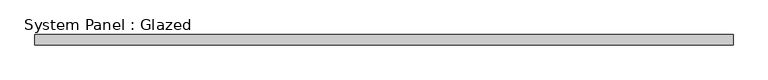
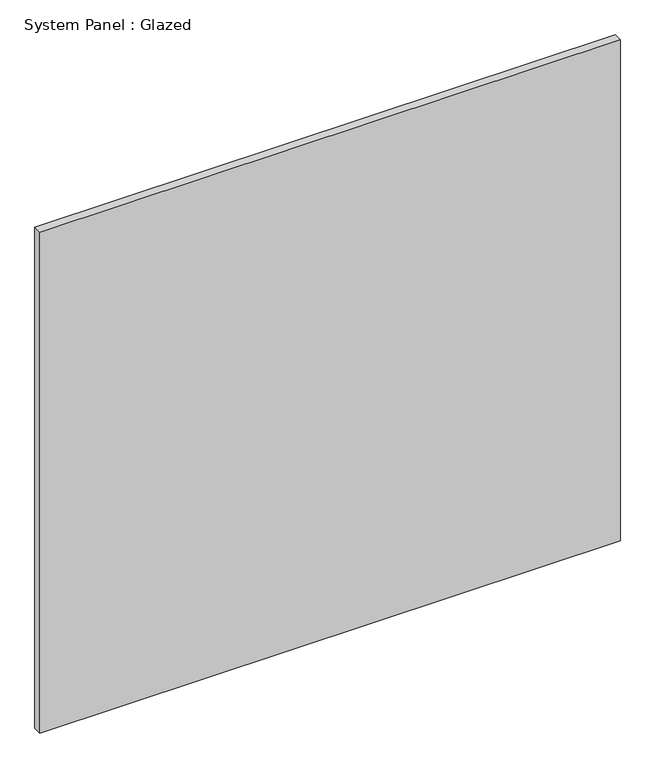
"""IFC4 building model written with IfcOpenShell, lengths in millimetres: plate geometry, System Panel : Glazed."""

import ifcopenshell
import ifcopenshell.guid

model = None  # the IFC model being written
_history = None  # IfcOwnerHistory: only IFC2X3 demands one
_inside = {}  # id of a spatial element -> (the spatial element, [elements in it])
_under = {}  # id of a project, library or spatial element -> (it, [spatial elements below it])
_declared = {}  # id of a project -> (the project, [libraries it declares])
_typed = {}  # id of a type object -> (the type object, [elements of that type])
_made_of = {}  # id of a material, layer set ... -> (it, [elements and type objects made of it])


def new_model(schema):
    """Start an empty IFC model of exactly this schema.

    Asked for "IFC4X3", IfcOpenShell would pick the latest addendum, in which some entities
    have other attributes; the version numbers below select the first issue.
    IFC2X3 requires an IfcOwnerHistory on every rooted entity: one is made here for all.
    """
    global model, _history
    if schema == "IFC4X3":
        model = ifcopenshell.file(schema_version=(4, 3, 0, 0))
    else:
        model = ifcopenshell.file(schema=schema)
    _inside.clear()
    _under.clear()
    _declared.clear()
    _typed.clear()
    _made_of.clear()
    _history = None
    if model.schema == "IFC2X3":
        org = make("IfcOrganization", Name="unknown")
        user = make(
            "IfcPersonAndOrganization",
            ThePerson=make("IfcPerson", FamilyName="unknown"),
            TheOrganization=org,
        )
        app = make(
            "IfcApplication",
            ApplicationDeveloper=org,
            Version="unknown",
            ApplicationFullName="unknown",
            ApplicationIdentifier="unknown",
        )
        _history = make(
            "IfcOwnerHistory",
            OwningUser=user,
            OwningApplication=app,
            ChangeAction="ADDED",
            CreationDate=0,
        )
    return model


def make(cls, **values):
    """One entity of the class cls with the attributes given. An attribute that is None is left unset."""
    return model.create_entity(
        cls, **{name: value for name, value in values.items() if value is not None}
    )


def rooted(cls, **values):
    """An entity with a GlobalId (a new one), such as an element, a storey or a relation."""
    return make(cls, GlobalId=ifcopenshell.guid.new(), OwnerHistory=_history, **values)


def si_unit(unit_type, name, prefix=None):
    """IfcSIUnit, for example si_unit("LENGTHUNIT", "METRE", prefix="MILLI")."""
    return make("IfcSIUnit", UnitType=unit_type, Prefix=prefix, Name=name)


def assignment(units):
    """IfcUnitAssignment: the units of a project."""
    return None if units is None else make("IfcUnitAssignment", Units=units)


def point(xyz):
    """IfcCartesianPoint."""
    return None if xyz is None else make("IfcCartesianPoint", Coordinates=xyz)


def direction(xyz):
    """IfcDirection."""
    return None if xyz is None else make("IfcDirection", DirectionRatios=xyz)


def frame(location, z_axis=None, x_axis=None):
    """IfcAxis2Placement3D, a coordinate frame: its origin and axes. An axis left out is left unset."""
    return make(
        "IfcAxis2Placement3D",
        Location=point(location),
        Axis=direction(z_axis),
        RefDirection=direction(x_axis),
    )


def origin():
    """The frame at (0, 0, 0) with its axes left unset."""
    return frame((0.0, 0.0, 0.0))


def origin_with_axes():
    """The frame at (0, 0, 0) with the z axis (0, 0, 1) and the x axis (1, 0, 0) written out."""
    return frame((0.0, 0.0, 0.0), z_axis=(0.0, 0.0, 1.0), x_axis=(1.0, 0.0, 0.0))


def place(relative_to, where):
    """IfcLocalPlacement: puts the frame where relative to a parent placement (None: the world)."""
    return make(
        "IfcLocalPlacement", PlacementRelTo=relative_to, RelativePlacement=where
    )


def context(
    kind, dimensions, precision=None, world=None, true_north=None, identifier=None
):
    """IfcGeometricRepresentationContext, for example the 3D "Model" context."""
    return make(
        "IfcGeometricRepresentationContext",
        ContextIdentifier=identifier,
        ContextType=kind,
        CoordinateSpaceDimension=dimensions,
        Precision=precision,
        WorldCoordinateSystem=world,
        TrueNorth=true_north,
    )


def project(units=None, contexts=None):
    """IfcProject with its units and contexts."""
    return rooted(
        "IfcProject",
        Name="project",
        RepresentationContexts=contexts,
        UnitsInContext=assignment(units),
    )


def spatial(cls, under=None, at=None, **own):
    """A site, building, storey or space (cls), placed at a placement, below another one or the project."""
    s = rooted(cls, ObjectPlacement=at, **own)
    if under is not None:
        _under.setdefault(under.id(), (under, []))[1].append(s)
    return s


def polyline(points):
    """IfcPolyline through the points."""
    return make("IfcPolyline", Points=[point(p) for p in points])


def outline(outer, holes=None, kind="AREA"):
    """IfcArbitraryClosedProfileDef: a profile drawn as a closed curve; with holes, ...WithVoids."""
    if holes is None:
        return make("IfcArbitraryClosedProfileDef", ProfileType=kind, OuterCurve=outer)
    return make(
        "IfcArbitraryProfileDefWithVoids",
        ProfileType=kind,
        OuterCurve=outer,
        InnerCurves=holes,
    )


def extrude(swept, where, along, depth):
    """IfcExtrudedAreaSolid: the profile swept, set in the frame where, extruded along a direction by depth."""
    return make(
        "IfcExtrudedAreaSolid",
        SweptArea=swept,
        Position=where,
        ExtrudedDirection=direction(along),
        Depth=depth,
    )


def shape(context_of_items, identifier, shape_type, items):
    """IfcShapeRepresentation: the items that make up one representation, for example the "Body"."""
    return make(
        "IfcShapeRepresentation",
        ContextOfItems=context_of_items,
        RepresentationIdentifier=identifier,
        RepresentationType=shape_type,
        Items=items,
    )


def source(mapping_origin, context_of_items, identifier, shape_type, items):
    """IfcRepresentationMap: a shape defined once, which mapped items show again and again."""
    return make(
        "IfcRepresentationMap",
        MappingOrigin=mapping_origin,
        MappedRepresentation=shape(context_of_items, identifier, shape_type, items),
    )


def transform(
    local_origin,
    x_axis=None,
    y_axis=None,
    z_axis=None,
    scale=None,
    scale2=None,
    scale3=None,
    uniform=True,
):
    """IfcCartesianTransformationOperator3D, or its non-uniform kind. x_axis, y_axis, z_axis: its Axis1, 2, 3."""
    if uniform:
        return make(
            "IfcCartesianTransformationOperator3D",
            Axis1=direction(x_axis),
            Axis2=direction(y_axis),
            LocalOrigin=point(local_origin),
            Scale=scale,
            Axis3=direction(z_axis),
        )
    return make(
        "IfcCartesianTransformationOperator3DnonUniform",
        Axis1=direction(x_axis),
        Axis2=direction(y_axis),
        LocalOrigin=point(local_origin),
        Scale=scale,
        Axis3=direction(z_axis),
        Scale2=scale2,
        Scale3=scale3,
    )


def mapped(mapping_source, mapping_target):
    """IfcMappedItem: shows the shape of a source again, moved by a transform."""
    return make(
        "IfcMappedItem", MappingSource=mapping_source, MappingTarget=mapping_target
    )


def made_of(thing, what):
    """Note that an element or type object is made of a material, layer set ...; save() writes the relation."""
    if what is not None:
        _made_of.setdefault(what.id(), (what, []))[1].append(thing)
    return thing


def element(
    cls,
    number,
    at=None,
    inside=None,
    cuts=None,
    type_object=None,
    material=None,
    context=None,
    identifier="Body",
    shape_type=None,
    held_by="IfcProductDefinitionShape",
    body=None,
    shapes=None,
    **own,
):
    """One element of the class cls, such as IfcWall. Its Tag is "e" and its number.

    at: its placement. inside: the storey or other place that contains it. cuts: it is an
    opening in that element (IfcRelVoidsElement). A single representation is given by context,
    identifier, shape_type and body (its items); several are given by shapes. held_by: the class
    of the entity that holds the representations. save() writes the other relations.
    """
    e = rooted(cls, Tag="e%d" % number, ObjectPlacement=at, **own)
    if body is not None:
        shapes = [shape(context, identifier, shape_type, body)]
    if shapes is not None:
        e.Representation = make(held_by, Representations=shapes)
    if inside is not None:
        _inside.setdefault(inside.id(), (inside, []))[1].append(e)
    if cuts is not None:
        rooted(
            "IfcRelVoidsElement", RelatingBuildingElement=cuts, RelatedOpeningElement=e
        )
    if type_object is not None:
        _typed.setdefault(type_object.id(), (type_object, []))[1].append(e)
    return made_of(e, material)


def aggregate(whole, parts):
    """IfcRelAggregates: a whole, such as a stair, and the parts it consists of."""
    return rooted("IfcRelAggregates", RelatingObject=whole, RelatedObjects=parts)


def save(model, path):
    """Write the relations noted so far, then the file.

    IfcRelAggregates (storeys below a building ...), IfcRelContainedInSpatialStructure (elements
    in a storey), IfcRelDefinesByType, IfcRelAssociatesMaterial and IfcRelDeclares: one each for
    every whole, place, type object, material and project.
    """
    for whole, parts in _under.values():
        aggregate(whole, parts)
    for where, things in _inside.values():
        rooted(
            "IfcRelContainedInSpatialStructure",
            RelatedElements=things,
            RelatingStructure=where,
        )
    for kind, things in _typed.values():
        rooted("IfcRelDefinesByType", RelatedObjects=things, RelatingType=kind)
    for what, things in _made_of.values():
        rooted("IfcRelAssociatesMaterial", RelatedObjects=things, RelatingMaterial=what)
    for by, libraries in _declared.values():
        rooted("IfcRelDeclares", RelatingContext=by, RelatedDefinitions=libraries)
    model.write(path)


def system_panel_glazed_22c1f233(model_context):
    return source(origin(), model_context, "Body", "SweptSolid", [
        extrude(outline(polyline([(866.7750114, 19.05), (-866.7750114, 19.05), (-866.7750114, 44.45), (866.7750114, 44.45), (866.7750114, 19.05)])), origin_with_axes(), (0.0, 0.0, 1.0), 1581.15),
    ])


if __name__ == "__main__":
    model = new_model("IFC4")
    model_context = context("Model", 3, world=origin())
    ifc_project = project(units=[si_unit("LENGTHUNIT", "METRE", prefix="MILLI")], contexts=[model_context])
    site = spatial("IfcSite", under=ifc_project)
    building = spatial("IfcBuilding", under=site)
    placement = place(None, origin())
    system_panel_glazed_shape = system_panel_glazed_22c1f233(model_context)
    element("IfcPlate", 1, ObjectType="System Panel : Glazed", at=placement, inside=building, context=model_context, shape_type="MappedRepresentation", body=[
        mapped(system_panel_glazed_shape, transform((0.0, 0.0, 0.0), x_axis=(1.0, 0.0, 0.0), y_axis=(0.0, 1.0, 0.0), z_axis=(0.0, 0.0, 1.0))),
    ])
    save(model, "model.ifc")

# Revit data of these elements
# Type "System Panel : Glazed"
#   Construction Type Id = "GSP4R"
#   Analytic Construction = "1/8 in Pilkington single glazing"
#   Visual Light Transmittance = 0.9
#   Solar Heat Gain Coefficient = 0.86
#   Heat Transfer Coefficient (U) = 1.18115 BTU/(h·ft²·°F)
#   Define Thermal Properties by = 1
# Element 1 (IfcPlate, "System Panel : Glazed")
#   Materials on its faces: "Glass"
# Materials
#   "Glass": class "Glass", colour RGB 0 128 192, transparency 0.75, Description = "Soda Lime Glass", Cost = 0
